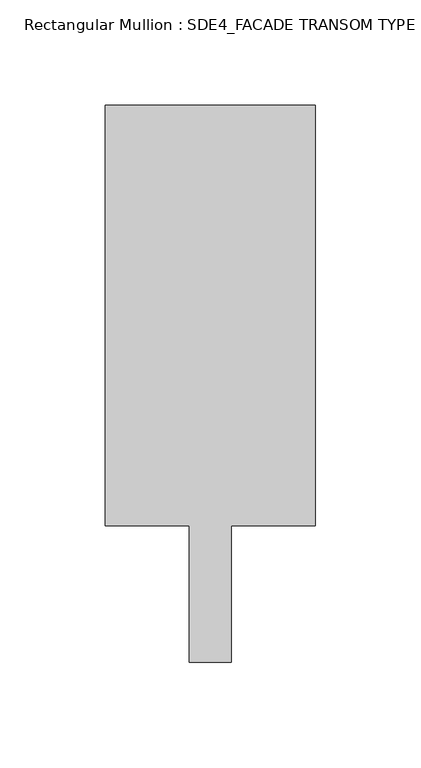
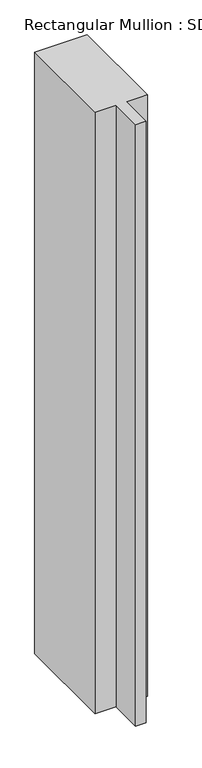
"""IFC4 building model written with IfcOpenShell, lengths in millimetres: member geometry, Rectangular Mullion : SDE4_FACADE TRANSOM TYPE 2."""

from ifc_helpers import new_model, si_unit, frame, origin, place, context, project, spatial, polyline, outline, extrude, source, transform, mapped, element, save


def rectangular_mullion_sde4_facade_transom_type_2_eb2d8785(model_context):
    return source(origin(), model_context, "Body", "SweptSolid", [
        extrude(outline(polyline([(50.0, 132.5), (50.0, -67.5), (10.0, -67.5), (10.0, -132.5), (-10.0, -132.5), (-10.0, -67.5), (-50.0, -67.5), (-50.0, 132.5), (50.0, 132.5)])), frame((0.0, 0.0, -1215.0), z_axis=(0.0, 0.0, 1.0), x_axis=(1.0, 0.0, 0.0)), (0.0, 0.0, 1.0), 1215.0),
    ])


if __name__ == "__main__":
    model = new_model("IFC4")
    model_context = context("Model", 3, world=origin())
    ifc_project = project(units=[si_unit("LENGTHUNIT", "METRE", prefix="MILLI")], contexts=[model_context])
    site = spatial("IfcSite", under=ifc_project)
    building = spatial("IfcBuilding", under=site)
    placement = place(None, origin())
    rectangular_mullion_sde4_facade_transom_type_2_shape = rectangular_mullion_sde4_facade_transom_type_2_eb2d8785(model_context)
    element("IfcMember", 1, ObjectType="Rectangular Mullion : SDE4_FACADE TRANSOM TYPE 2", at=placement, inside=building, context=model_context, shape_type="MappedRepresentation", body=[
        mapped(rectangular_mullion_sde4_facade_transom_type_2_shape, transform((0.0, 0.0, 0.0), x_axis=(1.0, 0.0, 0.0), y_axis=(0.0, 1.0, 0.0), z_axis=(0.0, 0.0, 1.0))),
    ])
    save(model, "model.ifc")

# Revit data of these elements
# Type "Rectangular Mullion : SDE4_FACADE TRANSOM TYPE 2"
#   built-in parameter 1007322 = 0.869423 (stored number, unit not read)
#   built-in parameter 1007321 = 0.164042 (stored number, unit not read)
#   built-in parameter 1007320 = 0.164042 (stored number, unit not read)
